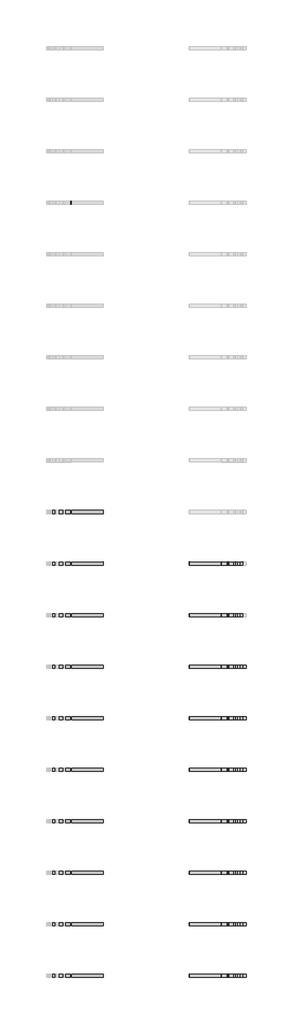
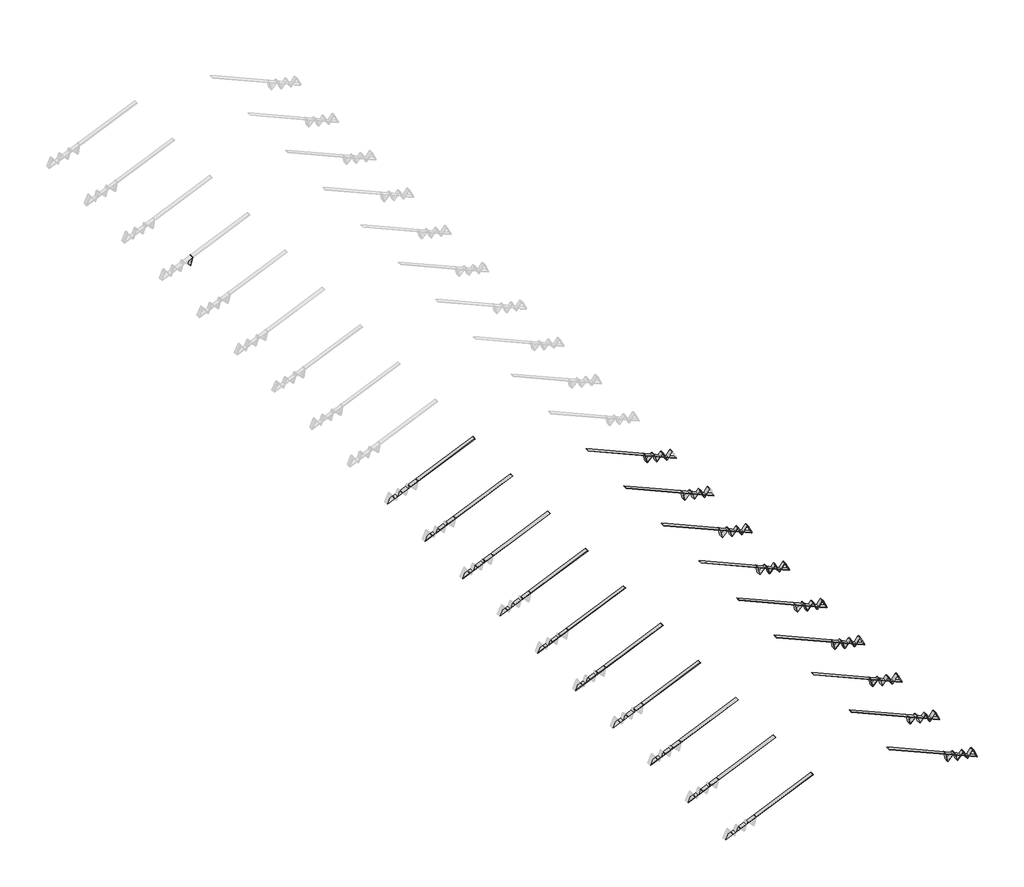
# One storey, part 2 of 4: 81 beams.
"""IFC4 building model written with IfcOpenShell, lengths in millimetres."""

import ifcopenshell
import ifcopenshell.guid

model = None  # the IFC model being written
_history = None  # IfcOwnerHistory: only IFC2X3 demands one
_inside = {}  # id of a spatial element -> (the spatial element, [elements in it])
_under = {}  # id of a project, library or spatial element -> (it, [spatial elements below it])
_declared = {}  # id of a project -> (the project, [libraries it declares])
_typed = {}  # id of a type object -> (the type object, [elements of that type])
_made_of = {}  # id of a material, layer set ... -> (it, [elements and type objects made of it])


def new_model(schema):
    """Start an empty IFC model of exactly this schema.

    Asked for "IFC4X3", IfcOpenShell would pick the latest addendum, in which some entities
    have other attributes; the version numbers below select the first issue.
    IFC2X3 requires an IfcOwnerHistory on every rooted entity: one is made here for all.
    """
    global model, _history
    if schema == "IFC4X3":
        model = ifcopenshell.file(schema_version=(4, 3, 0, 0))
    else:
        model = ifcopenshell.file(schema=schema)
    _inside.clear()
    _under.clear()
    _declared.clear()
    _typed.clear()
    _made_of.clear()
    _history = None
    if model.schema == "IFC2X3":
        org = make("IfcOrganization", Name="unknown")
        user = make(
            "IfcPersonAndOrganization",
            ThePerson=make("IfcPerson", FamilyName="unknown"),
            TheOrganization=org,
        )
        app = make(
            "IfcApplication",
            ApplicationDeveloper=org,
            Version="unknown",
            ApplicationFullName="unknown",
            ApplicationIdentifier="unknown",
        )
        _history = make(
            "IfcOwnerHistory",
            OwningUser=user,
            OwningApplication=app,
            ChangeAction="ADDED",
            CreationDate=0,
        )
    return model


def make(cls, **values):
    """One entity of the class cls with the attributes given. An attribute that is None is left unset."""
    return model.create_entity(
        cls, **{name: value for name, value in values.items() if value is not None}
    )


def rooted(cls, **values):
    """An entity with a GlobalId (a new one), such as an element, a storey or a relation."""
    return make(cls, GlobalId=ifcopenshell.guid.new(), OwnerHistory=_history, **values)


def si_unit(unit_type, name, prefix=None):
    """IfcSIUnit, for example si_unit("LENGTHUNIT", "METRE", prefix="MILLI")."""
    return make("IfcSIUnit", UnitType=unit_type, Prefix=prefix, Name=name)


def assignment(units):
    """IfcUnitAssignment: the units of a project."""
    return None if units is None else make("IfcUnitAssignment", Units=units)


def point(xyz):
    """IfcCartesianPoint."""
    return None if xyz is None else make("IfcCartesianPoint", Coordinates=xyz)


def direction(xyz):
    """IfcDirection."""
    return None if xyz is None else make("IfcDirection", DirectionRatios=xyz)


def frame(location, z_axis=None, x_axis=None):
    """IfcAxis2Placement3D, a coordinate frame: its origin and axes. An axis left out is left unset."""
    return make(
        "IfcAxis2Placement3D",
        Location=point(location),
        Axis=direction(z_axis),
        RefDirection=direction(x_axis),
    )


def frame_2d(location, x_axis=None):
    """IfcAxis2Placement2D, a coordinate frame in the plane: its origin and x axis."""
    return make(
        "IfcAxis2Placement2D", Location=point(location), RefDirection=direction(x_axis)
    )


def origin():
    """The frame at (0, 0, 0) with its axes left unset."""
    return frame((0.0, 0.0, 0.0))


def place(relative_to, where):
    """IfcLocalPlacement: puts the frame where relative to a parent placement (None: the world)."""
    return make(
        "IfcLocalPlacement", PlacementRelTo=relative_to, RelativePlacement=where
    )


def context(
    kind, dimensions, precision=None, world=None, true_north=None, identifier=None
):
    """IfcGeometricRepresentationContext, for example the 3D "Model" context."""
    return make(
        "IfcGeometricRepresentationContext",
        ContextIdentifier=identifier,
        ContextType=kind,
        CoordinateSpaceDimension=dimensions,
        Precision=precision,
        WorldCoordinateSystem=world,
        TrueNorth=true_north,
    )


def project(units=None, contexts=None):
    """IfcProject with its units and contexts."""
    return rooted(
        "IfcProject",
        Name="project",
        RepresentationContexts=contexts,
        UnitsInContext=assignment(units),
    )


def spatial(cls, under=None, at=None, **own):
    """A site, building, storey or space (cls), placed at a placement, below another one or the project."""
    s = rooted(cls, ObjectPlacement=at, **own)
    if under is not None:
        _under.setdefault(under.id(), (under, []))[1].append(s)
    return s


def polyline(points):
    """IfcPolyline through the points."""
    return make("IfcPolyline", Points=[point(p) for p in points])


def circle_curve(where, radius):
    """IfcCircle in the frame where."""
    return make("IfcCircle", Position=where, Radius=radius)


def trimmed(basis, trim1, trim2, sense, master):
    """IfcTrimmedCurve: the piece of a basis curve between two trims."""
    return make(
        "IfcTrimmedCurve",
        BasisCurve=basis,
        Trim1=trim1,
        Trim2=trim2,
        SenseAgreement=sense,
        MasterRepresentation=master,
    )


def segment(curve, same_sense, transition):
    """IfcCompositeCurveSegment."""
    return make(
        "IfcCompositeCurveSegment",
        Transition=transition,
        SameSense=same_sense,
        ParentCurve=curve,
    )


def composite_curve(segments, self_intersect=None):
    """IfcCompositeCurve: segments joined end to end."""
    return make("IfcCompositeCurve", Segments=segments, SelfIntersect=self_intersect)


def outline(outer, holes=None, kind="AREA"):
    """IfcArbitraryClosedProfileDef: a profile drawn as a closed curve; with holes, ...WithVoids."""
    if holes is None:
        return make("IfcArbitraryClosedProfileDef", ProfileType=kind, OuterCurve=outer)
    return make(
        "IfcArbitraryProfileDefWithVoids",
        ProfileType=kind,
        OuterCurve=outer,
        InnerCurves=holes,
    )


def extrude(swept, where, along, depth):
    """IfcExtrudedAreaSolid: the profile swept, set in the frame where, extruded along a direction by depth."""
    return make(
        "IfcExtrudedAreaSolid",
        SweptArea=swept,
        Position=where,
        ExtrudedDirection=direction(along),
        Depth=depth,
    )


def shape(context_of_items, identifier, shape_type, items):
    """IfcShapeRepresentation: the items that make up one representation, for example the "Body"."""
    return make(
        "IfcShapeRepresentation",
        ContextOfItems=context_of_items,
        RepresentationIdentifier=identifier,
        RepresentationType=shape_type,
        Items=items,
    )


def source(mapping_origin, context_of_items, identifier, shape_type, items):
    """IfcRepresentationMap: a shape defined once, which mapped items show again and again."""
    return make(
        "IfcRepresentationMap",
        MappingOrigin=mapping_origin,
        MappedRepresentation=shape(context_of_items, identifier, shape_type, items),
    )


def transform(
    local_origin,
    x_axis=None,
    y_axis=None,
    z_axis=None,
    scale=None,
    scale2=None,
    scale3=None,
    uniform=True,
):
    """IfcCartesianTransformationOperator3D, or its non-uniform kind. x_axis, y_axis, z_axis: its Axis1, 2, 3."""
    if uniform:
        return make(
            "IfcCartesianTransformationOperator3D",
            Axis1=direction(x_axis),
            Axis2=direction(y_axis),
            LocalOrigin=point(local_origin),
            Scale=scale,
            Axis3=direction(z_axis),
        )
    return make(
        "IfcCartesianTransformationOperator3DnonUniform",
        Axis1=direction(x_axis),
        Axis2=direction(y_axis),
        LocalOrigin=point(local_origin),
        Scale=scale,
        Axis3=direction(z_axis),
        Scale2=scale2,
        Scale3=scale3,
    )


def mapped(mapping_source, mapping_target):
    """IfcMappedItem: shows the shape of a source again, moved by a transform."""
    return make(
        "IfcMappedItem", MappingSource=mapping_source, MappingTarget=mapping_target
    )


def made_of(thing, what):
    """Note that an element or type object is made of a material, layer set ...; save() writes the relation."""
    if what is not None:
        _made_of.setdefault(what.id(), (what, []))[1].append(thing)
    return thing


def element(
    cls,
    number,
    at=None,
    inside=None,
    cuts=None,
    type_object=None,
    material=None,
    context=None,
    identifier="Body",
    shape_type=None,
    held_by="IfcProductDefinitionShape",
    body=None,
    shapes=None,
    **own,
):
    """One element of the class cls, such as IfcWall. Its Tag is "e" and its number.

    at: its placement. inside: the storey or other place that contains it. cuts: it is an
    opening in that element (IfcRelVoidsElement). A single representation is given by context,
    identifier, shape_type and body (its items); several are given by shapes. held_by: the class
    of the entity that holds the representations. save() writes the other relations.
    """
    e = rooted(cls, Tag="e%d" % number, ObjectPlacement=at, **own)
    if body is not None:
        shapes = [shape(context, identifier, shape_type, body)]
    if shapes is not None:
        e.Representation = make(held_by, Representations=shapes)
    if inside is not None:
        _inside.setdefault(inside.id(), (inside, []))[1].append(e)
    if cuts is not None:
        rooted(
            "IfcRelVoidsElement", RelatingBuildingElement=cuts, RelatedOpeningElement=e
        )
    if type_object is not None:
        _typed.setdefault(type_object.id(), (type_object, []))[1].append(e)
    return made_of(e, material)


def aggregate(whole, parts):
    """IfcRelAggregates: a whole, such as a stair, and the parts it consists of."""
    return rooted("IfcRelAggregates", RelatingObject=whole, RelatedObjects=parts)


def save(model, path):
    """Write the relations noted so far, then the file.

    IfcRelAggregates (storeys below a building ...), IfcRelContainedInSpatialStructure (elements
    in a storey), IfcRelDefinesByType, IfcRelAssociatesMaterial and IfcRelDeclares: one each for
    every whole, place, type object, material and project.
    """
    for whole, parts in _under.values():
        aggregate(whole, parts)
    for where, things in _inside.values():
        rooted(
            "IfcRelContainedInSpatialStructure",
            RelatedElements=things,
            RelatingStructure=where,
        )
    for kind, things in _typed.values():
        rooted("IfcRelDefinesByType", RelatedObjects=things, RelatingType=kind)
    for what, things in _made_of.values():
        rooted("IfcRelAssociatesMaterial", RelatedObjects=things, RelatingMaterial=what)
    for by, libraries in _declared.values():
        rooted("IfcRelDeclares", RelatingContext=by, RelatedDefinitions=libraries)
    model.write(path)


def placa_diagonal_af2a04a3(model_context):
    return source(origin(), model_context, "Body", "SweptSolid", [
        extrude(outline(polyline([(165.1705216, 75.0), (165.1705216, -75.0), (-165.4962729, -75.0), (-165.4962729, 75.0), (165.1705216, 75.0)])), frame((0.0, 0.0, -4.0), z_axis=(0.0, 0.0, 1.0), x_axis=(1.0, 0.0, 0.0)), (0.0, 0.0, 1.0), 8.0),
    ])


def placa_diagonal_6d03bdc5(model_context):
    return source(origin(), model_context, "Body", "SweptSolid", [
        extrude(outline(polyline([(191.209825, 75.0), (191.209825, -75.0), (-166.9394885, -75.0), (-166.9394885, 75.0), (191.209825, 75.0)])), frame((0.0, 0.0, -4.0), z_axis=(0.0, 0.0, 1.0), x_axis=(1.0, 0.0, 0.0)), (0.0, 0.0, 1.0), 8.0),
    ])


def placa_diagonal_30fa4039(model_context):
    return source(origin(), model_context, "Body", "SweptSolid", [
        extrude(outline(polyline([(167.0675386, 75.0), (167.0675386, -75.0), (-167.4240159, -75.0), (-167.4240159, 75.0), (167.0675386, 75.0)])), frame((0.0, 0.0, -4.0), z_axis=(0.0, 0.0, 1.0), x_axis=(1.0, 0.0, 0.0)), (0.0, 0.0, 1.0), 8.0),
    ])


def placa_diagonal_ded414cc(model_context):
    return source(origin(), model_context, "Body", "SweptSolid", [
        extrude(outline(polyline([(167.4240165, 75.0), (167.4240165, -75.0), (-167.0675392, -75.0), (-167.0675392, 75.0), (167.4240165, 75.0)])), frame((0.0, 0.0, -4.0), z_axis=(0.0, 0.0, 1.0), x_axis=(1.0, 0.0, 0.0)), (0.0, 0.0, 1.0), 8.0),
    ])


def placa_diagonal_4690b74a(model_context):
    return source(origin(), model_context, "Body", "SweptSolid", [
        extrude(outline(polyline([(167.0675389, 75.0), (167.0675389, -75.0), (-167.4240162, -75.0), (-167.4240162, 75.0), (167.0675389, 75.0)])), frame((0.0, 0.0, -4.0), z_axis=(0.0, 0.0, 1.0), x_axis=(1.0, 0.0, 0.0)), (0.0, 0.0, 1.0), 8.0),
    ])


def placa_diagonal_aaf0c3b6(model_context):
    return source(origin(), model_context, "Body", "SweptSolid", [
        extrude(outline(polyline([(167.4240163, 75.0), (167.4240163, -75.0), (-167.067539, -75.0), (-167.067539, 75.0), (167.4240163, 75.0)])), frame((0.0, 0.0, -4.0), z_axis=(0.0, 0.0, 1.0), x_axis=(1.0, 0.0, 0.0)), (0.0, 0.0, 1.0), 8.0),
    ])


model = new_model("IFC4")

# Units and contexts
model_context = context("Model", 3, world=origin())
ifc_project = project(units=[si_unit("LENGTHUNIT", "METRE", prefix="MILLI")], contexts=[model_context])

# Site, building, storey
site = spatial("IfcSite", under=ifc_project)
building = spatial("IfcBuilding", under=site)
storey = spatial("IfcBuildingStorey", under=building, Name="Nível 4", Elevation=48165.0)

# Beams
placement = place(None, origin())
element("IfcBeam", 1, ObjectType="Placa : banzo", at=placement, inside=storey, context=model_context, shape_type="SweptSolid", body=[
    extrude(outline(composite_curve([segment(polyline([(48158.5516223, 8114.9704041), (48174.5198715, 8115.9778843)]), True, "CONTINUOUS"), segment(trimmed(circle_curve(frame_2d((53506.1312788, 8452.3636953)), 5342.2126139), [point((48174.5198715, 8115.9778843))], [point((49646.1683419, 4759.1372282))], True, "CARTESIAN"), True, "CONTINUOUS"), segment(polyline([(49646.1683419, 4759.1372282), (49634.6077, 4748.0759643)]), True, "CONTINUOUS"), segment(trimmed(circle_curve(frame_2d((53506.1312788, 8452.3636953)), 5358.2126139), [point((49634.6077, 4748.0759643))], [point((48158.5516223, 8114.9704041))], False, "CARTESIAN"), True, "CONTINUOUS")], self_intersect=False)), frame((0.0, -39678.5623634, 0.0), z_axis=(0.0, 1.0, 0.0), x_axis=(0.0, 0.0, 1.0)), (0.0, 0.0, 1.0), 150.0),
])
element("IfcBeam", 2, ObjectType="Placa : banzo", at=placement, inside=storey, context=model_context, shape_type="SweptSolid", body=[
    extrude(outline(composite_curve([segment(polyline([(49634.6077, 1843.8240278), (49646.1683419, 1832.762764)]), True, "CONTINUOUS"), segment(trimmed(circle_curve(frame_2d((53506.1312788, -1860.4637031)), 5342.2126139), [point((49646.1683419, 1832.762764))], [point((48174.5198715, -1524.0778921))], True, "CARTESIAN"), True, "CONTINUOUS"), segment(polyline([(48174.5198715, -1524.0778921), (48158.5516223, -1523.070412)]), True, "CONTINUOUS"), segment(trimmed(circle_curve(frame_2d((53506.1312788, -1860.4637031)), 5358.2126139), [point((48158.5516223, -1523.070412))], [point((49634.6077, 1843.8240278))], False, "CARTESIAN"), True, "CONTINUOUS")], self_intersect=False)), frame((0.0, -39678.5623634, 0.0), z_axis=(0.0, 1.0, 0.0), x_axis=(0.0, 0.0, 1.0)), (0.0, 0.0, 1.0), 150.0),
])
element("IfcBeam", 3, ObjectType="Placa : banzo", at=placement, inside=storey, context=model_context, shape_type="SweptSolid", body=[
    extrude(outline(composite_curve([segment(polyline([(49634.6077, 1843.8240278), (49646.1683419, 1832.762764)]), True, "CONTINUOUS"), segment(trimmed(circle_curve(frame_2d((53506.1312788, -1860.4637031)), 5342.2126139), [point((49646.1683419, 1832.762764))], [point((48174.5198715, -1524.0778921))], True, "CARTESIAN"), True, "CONTINUOUS"), segment(polyline([(48174.5198715, -1524.0778921), (48158.5516223, -1523.070412)]), True, "CONTINUOUS"), segment(trimmed(circle_curve(frame_2d((53506.1312788, -1860.4637031)), 5358.2126139), [point((48158.5516223, -1523.070412))], [point((49634.6077, 1843.8240278))], False, "CARTESIAN"), True, "CONTINUOUS")], self_intersect=False)), frame((0.0, -17178.5623634, 0.0), z_axis=(0.0, 1.0, 0.0), x_axis=(0.0, 0.0, 1.0)), (0.0, 0.0, 1.0), 150.0),
])
element("IfcBeam", 4, ObjectType="Placa : banzo", at=placement, inside=storey, context=model_context, shape_type="SweptSolid", body=[
    extrude(outline(composite_curve([segment(polyline([(48158.5516223, 8114.9704041), (48174.5198715, 8115.9778843)]), True, "CONTINUOUS"), segment(trimmed(circle_curve(frame_2d((53506.1312788, 8452.3636953)), 5342.2126139), [point((48174.5198715, 8115.9778843))], [point((49646.1683419, 4759.1372282))], True, "CARTESIAN"), True, "CONTINUOUS"), segment(polyline([(49646.1683419, 4759.1372282), (49634.6077, 4748.0759643)]), True, "CONTINUOUS"), segment(trimmed(circle_curve(frame_2d((53506.1312788, 8452.3636953)), 5358.2126139), [point((49634.6077, 4748.0759643))], [point((48158.5516223, 8114.9704041))], False, "CARTESIAN"), True, "CONTINUOUS")], self_intersect=False)), frame((0.0, -19678.5623634, 0.0), z_axis=(0.0, 1.0, 0.0), x_axis=(0.0, 0.0, 1.0)), (0.0, 0.0, 1.0), 150.0),
])
element("IfcBeam", 5, ObjectType="Placa : banzo", at=placement, inside=storey, context=model_context, shape_type="SweptSolid", body=[
    extrude(outline(composite_curve([segment(polyline([(49634.6077, 1843.8240278), (49646.1683419, 1832.762764)]), True, "CONTINUOUS"), segment(trimmed(circle_curve(frame_2d((53506.1312788, -1860.4637031)), 5342.2126139), [point((49646.1683419, 1832.762764))], [point((48174.5198715, -1524.0778921))], True, "CARTESIAN"), True, "CONTINUOUS"), segment(polyline([(48174.5198715, -1524.0778921), (48158.5516223, -1523.070412)]), True, "CONTINUOUS"), segment(trimmed(circle_curve(frame_2d((53506.1312788, -1860.4637031)), 5358.2126139), [point((48158.5516223, -1523.070412))], [point((49634.6077, 1843.8240278))], False, "CARTESIAN"), True, "CONTINUOUS")], self_intersect=False)), frame((0.0, -19678.5623634, 0.0), z_axis=(0.0, 1.0, 0.0), x_axis=(0.0, 0.0, 1.0)), (0.0, 0.0, 1.0), 150.0),
])
element("IfcBeam", 6, ObjectType="Placa : banzo", at=placement, inside=storey, context=model_context, shape_type="SweptSolid", body=[
    extrude(outline(composite_curve([segment(polyline([(48158.5516223, 8114.9704041), (48174.5198715, 8115.9778843)]), True, "CONTINUOUS"), segment(trimmed(circle_curve(frame_2d((53506.1312788, 8452.3636953)), 5342.2126139), [point((48174.5198715, 8115.9778843))], [point((49646.1683419, 4759.1372282))], True, "CARTESIAN"), True, "CONTINUOUS"), segment(polyline([(49646.1683419, 4759.1372282), (49634.6077, 4748.0759643)]), True, "CONTINUOUS"), segment(trimmed(circle_curve(frame_2d((53506.1312788, 8452.3636953)), 5358.2126139), [point((49634.6077, 4748.0759643))], [point((48158.5516223, 8114.9704041))], False, "CARTESIAN"), True, "CONTINUOUS")], self_intersect=False)), frame((0.0, -22178.5623634, 0.0), z_axis=(0.0, 1.0, 0.0), x_axis=(0.0, 0.0, 1.0)), (0.0, 0.0, 1.0), 150.0),
])
element("IfcBeam", 7, ObjectType="Placa : banzo", at=placement, inside=storey, context=model_context, shape_type="SweptSolid", body=[
    extrude(outline(composite_curve([segment(polyline([(49634.6077, 1843.8240278), (49646.1683419, 1832.762764)]), True, "CONTINUOUS"), segment(trimmed(circle_curve(frame_2d((53506.1312788, -1860.4637031)), 5342.2126139), [point((49646.1683419, 1832.762764))], [point((48174.5198715, -1524.0778921))], True, "CARTESIAN"), True, "CONTINUOUS"), segment(polyline([(48174.5198715, -1524.0778921), (48158.5516223, -1523.070412)]), True, "CONTINUOUS"), segment(trimmed(circle_curve(frame_2d((53506.1312788, -1860.4637031)), 5358.2126139), [point((48158.5516223, -1523.070412))], [point((49634.6077, 1843.8240278))], False, "CARTESIAN"), True, "CONTINUOUS")], self_intersect=False)), frame((0.0, -22178.5623634, 0.0), z_axis=(0.0, 1.0, 0.0), x_axis=(0.0, 0.0, 1.0)), (0.0, 0.0, 1.0), 150.0),
])
element("IfcBeam", 8, ObjectType="Placa : banzo", at=placement, inside=storey, context=model_context, shape_type="SweptSolid", body=[
    extrude(outline(composite_curve([segment(polyline([(48158.5516223, 8114.9704041), (48174.5198715, 8115.9778843)]), True, "CONTINUOUS"), segment(trimmed(circle_curve(frame_2d((53506.1312788, 8452.3636953)), 5342.2126139), [point((48174.5198715, 8115.9778843))], [point((49646.1683419, 4759.1372282))], True, "CARTESIAN"), True, "CONTINUOUS"), segment(polyline([(49646.1683419, 4759.1372282), (49634.6077, 4748.0759643)]), True, "CONTINUOUS"), segment(trimmed(circle_curve(frame_2d((53506.1312788, 8452.3636953)), 5358.2126139), [point((49634.6077, 4748.0759643))], [point((48158.5516223, 8114.9704041))], False, "CARTESIAN"), True, "CONTINUOUS")], self_intersect=False)), frame((0.0, -24678.5623634, 0.0), z_axis=(0.0, 1.0, 0.0), x_axis=(0.0, 0.0, 1.0)), (0.0, 0.0, 1.0), 150.0),
])
element("IfcBeam", 9, ObjectType="Placa : banzo", at=placement, inside=storey, context=model_context, shape_type="SweptSolid", body=[
    extrude(outline(composite_curve([segment(polyline([(49634.6077, 1843.8240278), (49646.1683419, 1832.762764)]), True, "CONTINUOUS"), segment(trimmed(circle_curve(frame_2d((53506.1312788, -1860.4637031)), 5342.2126139), [point((49646.1683419, 1832.762764))], [point((48174.5198715, -1524.0778921))], True, "CARTESIAN"), True, "CONTINUOUS"), segment(polyline([(48174.5198715, -1524.0778921), (48158.5516223, -1523.070412)]), True, "CONTINUOUS"), segment(trimmed(circle_curve(frame_2d((53506.1312788, -1860.4637031)), 5358.2126139), [point((48158.5516223, -1523.070412))], [point((49634.6077, 1843.8240278))], False, "CARTESIAN"), True, "CONTINUOUS")], self_intersect=False)), frame((0.0, -24678.5623634, 0.0), z_axis=(0.0, 1.0, 0.0), x_axis=(0.0, 0.0, 1.0)), (0.0, 0.0, 1.0), 150.0),
])
element("IfcBeam", 10, ObjectType="Placa : banzo", at=placement, inside=storey, context=model_context, shape_type="SweptSolid", body=[
    extrude(outline(composite_curve([segment(polyline([(48158.5516223, 8114.9704041), (48174.5198715, 8115.9778843)]), True, "CONTINUOUS"), segment(trimmed(circle_curve(frame_2d((53506.1312788, 8452.3636953)), 5342.2126139), [point((48174.5198715, 8115.9778843))], [point((49646.1683419, 4759.1372282))], True, "CARTESIAN"), True, "CONTINUOUS"), segment(polyline([(49646.1683419, 4759.1372282), (49634.6077, 4748.0759643)]), True, "CONTINUOUS"), segment(trimmed(circle_curve(frame_2d((53506.1312788, 8452.3636953)), 5358.2126139), [point((49634.6077, 4748.0759643))], [point((48158.5516223, 8114.9704041))], False, "CARTESIAN"), True, "CONTINUOUS")], self_intersect=False)), frame((0.0, -27178.5623634, 0.0), z_axis=(0.0, 1.0, 0.0), x_axis=(0.0, 0.0, 1.0)), (0.0, 0.0, 1.0), 150.0),
])
element("IfcBeam", 11, ObjectType="Placa : banzo", at=placement, inside=storey, context=model_context, shape_type="SweptSolid", body=[
    extrude(outline(composite_curve([segment(polyline([(49634.6077, 1843.8240278), (49646.1683419, 1832.762764)]), True, "CONTINUOUS"), segment(trimmed(circle_curve(frame_2d((53506.1312788, -1860.4637031)), 5342.2126139), [point((49646.1683419, 1832.762764))], [point((48174.5198715, -1524.0778921))], True, "CARTESIAN"), True, "CONTINUOUS"), segment(polyline([(48174.5198715, -1524.0778921), (48158.5516223, -1523.070412)]), True, "CONTINUOUS"), segment(trimmed(circle_curve(frame_2d((53506.1312788, -1860.4637031)), 5358.2126139), [point((48158.5516223, -1523.070412))], [point((49634.6077, 1843.8240278))], False, "CARTESIAN"), True, "CONTINUOUS")], self_intersect=False)), frame((0.0, -27178.5623634, 0.0), z_axis=(0.0, 1.0, 0.0), x_axis=(0.0, 0.0, 1.0)), (0.0, 0.0, 1.0), 150.0),
])
element("IfcBeam", 12, ObjectType="Placa : banzo", at=placement, inside=storey, context=model_context, shape_type="SweptSolid", body=[
    extrude(outline(composite_curve([segment(polyline([(48158.5516223, 8114.9704041), (48174.5198715, 8115.9778843)]), True, "CONTINUOUS"), segment(trimmed(circle_curve(frame_2d((53506.1312788, 8452.3636953)), 5342.2126139), [point((48174.5198715, 8115.9778843))], [point((49646.1683419, 4759.1372282))], True, "CARTESIAN"), True, "CONTINUOUS"), segment(polyline([(49646.1683419, 4759.1372282), (49634.6077, 4748.0759643)]), True, "CONTINUOUS"), segment(trimmed(circle_curve(frame_2d((53506.1312788, 8452.3636953)), 5358.2126139), [point((49634.6077, 4748.0759643))], [point((48158.5516223, 8114.9704041))], False, "CARTESIAN"), True, "CONTINUOUS")], self_intersect=False)), frame((0.0, -29678.5623634, 0.0), z_axis=(0.0, 1.0, 0.0), x_axis=(0.0, 0.0, 1.0)), (0.0, 0.0, 1.0), 150.0),
])
element("IfcBeam", 13, ObjectType="Placa : banzo", at=placement, inside=storey, context=model_context, shape_type="SweptSolid", body=[
    extrude(outline(composite_curve([segment(polyline([(49634.6077, 1843.8240278), (49646.1683419, 1832.762764)]), True, "CONTINUOUS"), segment(trimmed(circle_curve(frame_2d((53506.1312788, -1860.4637031)), 5342.2126139), [point((49646.1683419, 1832.762764))], [point((48174.5198715, -1524.0778921))], True, "CARTESIAN"), True, "CONTINUOUS"), segment(polyline([(48174.5198715, -1524.0778921), (48158.5516223, -1523.070412)]), True, "CONTINUOUS"), segment(trimmed(circle_curve(frame_2d((53506.1312788, -1860.4637031)), 5358.2126139), [point((48158.5516223, -1523.070412))], [point((49634.6077, 1843.8240278))], False, "CARTESIAN"), True, "CONTINUOUS")], self_intersect=False)), frame((0.0, -29678.5623634, 0.0), z_axis=(0.0, 1.0, 0.0), x_axis=(0.0, 0.0, 1.0)), (0.0, 0.0, 1.0), 150.0),
])
element("IfcBeam", 14, ObjectType="Placa : banzo", at=placement, inside=storey, context=model_context, shape_type="SweptSolid", body=[
    extrude(outline(composite_curve([segment(polyline([(48158.5516223, 8114.9704041), (48174.5198715, 8115.9778843)]), True, "CONTINUOUS"), segment(trimmed(circle_curve(frame_2d((53506.1312788, 8452.3636953)), 5342.2126139), [point((48174.5198715, 8115.9778843))], [point((49646.1683419, 4759.1372282))], True, "CARTESIAN"), True, "CONTINUOUS"), segment(polyline([(49646.1683419, 4759.1372282), (49634.6077, 4748.0759643)]), True, "CONTINUOUS"), segment(trimmed(circle_curve(frame_2d((53506.1312788, 8452.3636953)), 5358.2126139), [point((49634.6077, 4748.0759643))], [point((48158.5516223, 8114.9704041))], False, "CARTESIAN"), True, "CONTINUOUS")], self_intersect=False)), frame((0.0, -32178.5623634, 0.0), z_axis=(0.0, 1.0, 0.0), x_axis=(0.0, 0.0, 1.0)), (0.0, 0.0, 1.0), 150.0),
])
element("IfcBeam", 15, ObjectType="Placa : banzo", at=placement, inside=storey, context=model_context, shape_type="SweptSolid", body=[
    extrude(outline(composite_curve([segment(polyline([(49634.6077, 1843.8240278), (49646.1683419, 1832.762764)]), True, "CONTINUOUS"), segment(trimmed(circle_curve(frame_2d((53506.1312788, -1860.4637031)), 5342.2126139), [point((49646.1683419, 1832.762764))], [point((48174.5198715, -1524.0778921))], True, "CARTESIAN"), True, "CONTINUOUS"), segment(polyline([(48174.5198715, -1524.0778921), (48158.5516223, -1523.070412)]), True, "CONTINUOUS"), segment(trimmed(circle_curve(frame_2d((53506.1312788, -1860.4637031)), 5358.2126139), [point((48158.5516223, -1523.070412))], [point((49634.6077, 1843.8240278))], False, "CARTESIAN"), True, "CONTINUOUS")], self_intersect=False)), frame((0.0, -32178.5623634, 0.0), z_axis=(0.0, 1.0, 0.0), x_axis=(0.0, 0.0, 1.0)), (0.0, 0.0, 1.0), 150.0),
])
element("IfcBeam", 16, ObjectType="Placa : banzo", at=placement, inside=storey, context=model_context, shape_type="SweptSolid", body=[
    extrude(outline(composite_curve([segment(polyline([(48158.5516223, 8114.9704041), (48174.5198715, 8115.9778843)]), True, "CONTINUOUS"), segment(trimmed(circle_curve(frame_2d((53506.1312788, 8452.3636953)), 5342.2126139), [point((48174.5198715, 8115.9778843))], [point((49646.1683419, 4759.1372282))], True, "CARTESIAN"), True, "CONTINUOUS"), segment(polyline([(49646.1683419, 4759.1372282), (49634.6077, 4748.0759643)]), True, "CONTINUOUS"), segment(trimmed(circle_curve(frame_2d((53506.1312788, 8452.3636953)), 5358.2126139), [point((49634.6077, 4748.0759643))], [point((48158.5516223, 8114.9704041))], False, "CARTESIAN"), True, "CONTINUOUS")], self_intersect=False)), frame((0.0, -34678.5623634, 0.0), z_axis=(0.0, 1.0, 0.0), x_axis=(0.0, 0.0, 1.0)), (0.0, 0.0, 1.0), 150.0),
])
element("IfcBeam", 17, ObjectType="Placa : banzo", at=placement, inside=storey, context=model_context, shape_type="SweptSolid", body=[
    extrude(outline(composite_curve([segment(polyline([(49634.6077, 1843.8240278), (49646.1683419, 1832.762764)]), True, "CONTINUOUS"), segment(trimmed(circle_curve(frame_2d((53506.1312788, -1860.4637031)), 5342.2126139), [point((49646.1683419, 1832.762764))], [point((48174.5198715, -1524.0778921))], True, "CARTESIAN"), True, "CONTINUOUS"), segment(polyline([(48174.5198715, -1524.0778921), (48158.5516223, -1523.070412)]), True, "CONTINUOUS"), segment(trimmed(circle_curve(frame_2d((53506.1312788, -1860.4637031)), 5358.2126139), [point((48158.5516223, -1523.070412))], [point((49634.6077, 1843.8240278))], False, "CARTESIAN"), True, "CONTINUOUS")], self_intersect=False)), frame((0.0, -34678.5623634, 0.0), z_axis=(0.0, 1.0, 0.0), x_axis=(0.0, 0.0, 1.0)), (0.0, 0.0, 1.0), 150.0),
])
element("IfcBeam", 18, ObjectType="Placa : banzo", at=placement, inside=storey, context=model_context, shape_type="SweptSolid", body=[
    extrude(outline(composite_curve([segment(polyline([(48158.5516223, 8114.9704041), (48174.5198715, 8115.9778843)]), True, "CONTINUOUS"), segment(trimmed(circle_curve(frame_2d((53506.1312788, 8452.3636953)), 5342.2126139), [point((48174.5198715, 8115.9778843))], [point((49646.1683419, 4759.1372282))], True, "CARTESIAN"), True, "CONTINUOUS"), segment(polyline([(49646.1683419, 4759.1372282), (49634.6077, 4748.0759643)]), True, "CONTINUOUS"), segment(trimmed(circle_curve(frame_2d((53506.1312788, 8452.3636953)), 5358.2126139), [point((49634.6077, 4748.0759643))], [point((48158.5516223, 8114.9704041))], False, "CARTESIAN"), True, "CONTINUOUS")], self_intersect=False)), frame((0.0, -37178.5623634, 0.0), z_axis=(0.0, 1.0, 0.0), x_axis=(0.0, 0.0, 1.0)), (0.0, 0.0, 1.0), 150.0),
])
element("IfcBeam", 19, ObjectType="Placa : banzo", at=placement, inside=storey, context=model_context, shape_type="SweptSolid", body=[
    extrude(outline(composite_curve([segment(polyline([(49634.6077, 1843.8240278), (49646.1683419, 1832.762764)]), True, "CONTINUOUS"), segment(trimmed(circle_curve(frame_2d((53506.1312788, -1860.4637031)), 5342.2126139), [point((49646.1683419, 1832.762764))], [point((48174.5198715, -1524.0778921))], True, "CARTESIAN"), True, "CONTINUOUS"), segment(polyline([(48174.5198715, -1524.0778921), (48158.5516223, -1523.070412)]), True, "CONTINUOUS"), segment(trimmed(circle_curve(frame_2d((53506.1312788, -1860.4637031)), 5358.2126139), [point((48158.5516223, -1523.070412))], [point((49634.6077, 1843.8240278))], False, "CARTESIAN"), True, "CONTINUOUS")], self_intersect=False)), frame((0.0, -37178.5623634, 0.0), z_axis=(0.0, 1.0, 0.0), x_axis=(0.0, 0.0, 1.0)), (0.0, 0.0, 1.0), 150.0),
])
placa_diagonal_shape = placa_diagonal_af2a04a3(model_context)
element("IfcBeam", 20, ObjectType="Placa : diagonal", at=placement, inside=storey, context=model_context, shape_type="MappedRepresentation", body=[
    mapped(placa_diagonal_shape, transform((-392.7303205, -2103.5623634, 48535.8666224), x_axis=(0.20085127706480188, 0.0, 0.9796217456250337), y_axis=(0.0, -1.0, 0.0), z_axis=(0.9796217456250337, 0.0, -0.20085127706480188))),
])
placa_diagonal_2_shape = placa_diagonal_6d03bdc5(model_context)
element("IfcBeam", 21, ObjectType="Placa : diagonal", at=placement, inside=storey, context=model_context, shape_type="MappedRepresentation", body=[
    mapped(placa_diagonal_2_shape, transform((8059.7198757, -39603.5623634, 48338.6280973), x_axis=(0.4189773842608123, 0.0, -0.9079966693099526), y_axis=(0.0, -1.0, 0.0), z_axis=(-0.9079966693099526, 0.0, -0.4189773842608123))),
])
element("IfcBeam", 22, ObjectType="Placa : diagonal", at=placement, inside=storey, context=model_context, shape_type="MappedRepresentation", body=[
    mapped(placa_diagonal_2_shape, transform((8059.7198757, -24603.5623634, 48338.6280973), x_axis=(0.4189773842608123, 0.0, -0.9079966693099526), y_axis=(0.0, -1.0, 0.0), z_axis=(-0.9079966693099526, 0.0, -0.4189773842608123))),
])
element("IfcBeam", 23, ObjectType="Placa : diagonal", at=placement, inside=storey, context=model_context, shape_type="MappedRepresentation", body=[
    mapped(placa_diagonal_2_shape, transform((8059.7198757, -27103.5623634, 48338.6280973), x_axis=(0.4189773842608123, 0.0, -0.9079966693099526), y_axis=(0.0, -1.0, 0.0), z_axis=(-0.9079966693099526, 0.0, -0.4189773842608123))),
])
element("IfcBeam", 24, ObjectType="Placa : diagonal", at=placement, inside=storey, context=model_context, shape_type="MappedRepresentation", body=[
    mapped(placa_diagonal_2_shape, transform((8059.7198757, -29603.5623634, 48338.6280973), x_axis=(0.4189773842608123, 0.0, -0.9079966693099526), y_axis=(0.0, -1.0, 0.0), z_axis=(-0.9079966693099526, 0.0, -0.4189773842608123))),
])
element("IfcBeam", 25, ObjectType="Placa : diagonal", at=placement, inside=storey, context=model_context, shape_type="MappedRepresentation", body=[
    mapped(placa_diagonal_2_shape, transform((8059.7198757, -32103.5623634, 48338.6280973), x_axis=(0.4189773842608123, 0.0, -0.9079966693099526), y_axis=(0.0, -1.0, 0.0), z_axis=(-0.9079966693099526, 0.0, -0.4189773842608123))),
])
element("IfcBeam", 26, ObjectType="Placa : diagonal", at=placement, inside=storey, context=model_context, shape_type="MappedRepresentation", body=[
    mapped(placa_diagonal_2_shape, transform((8059.7198757, -34603.5623634, 48338.6280973), x_axis=(0.4189773842608123, 0.0, -0.9079966693099526), y_axis=(0.0, -1.0, 0.0), z_axis=(-0.9079966693099526, 0.0, -0.4189773842608123))),
])
element("IfcBeam", 27, ObjectType="Placa : diagonal", at=placement, inside=storey, context=model_context, shape_type="MappedRepresentation", body=[
    mapped(placa_diagonal_2_shape, transform((8059.7198757, -37103.5623634, 48338.6280973), x_axis=(0.4189773842608123, 0.0, -0.9079966693099526), y_axis=(0.0, -1.0, 0.0), z_axis=(-0.9079966693099526, 0.0, -0.4189773842608123))),
])
placa_diagonal_3_shape = placa_diagonal_30fa4039(model_context)
element("IfcBeam", 28, ObjectType="Placa : diagonal", at=placement, inside=storey, context=model_context, shape_type="MappedRepresentation", body=[
    mapped(placa_diagonal_3_shape, transform((7867.9931921, -39603.5623634, 48356.8132581), x_axis=(0.5832804616623758, 0.0, 0.8122708310920229), y_axis=(0.0, -1.0, 0.0), z_axis=(0.8122708310920229, 0.0, -0.5832804616623758))),
])
element("IfcBeam", 29, ObjectType="Placa : diagonal", at=placement, inside=storey, context=model_context, shape_type="MappedRepresentation", body=[
    mapped(placa_diagonal_3_shape, transform((7867.9931921, -19603.5623634, 48356.8132581), x_axis=(0.5832804616623758, 0.0, 0.8122708310920229), y_axis=(0.0, -1.0, 0.0), z_axis=(0.8122708310920229, 0.0, -0.5832804616623758))),
])
element("IfcBeam", 30, ObjectType="Placa : diagonal", at=placement, inside=storey, context=model_context, shape_type="MappedRepresentation", body=[
    mapped(placa_diagonal_3_shape, transform((7867.9931921, -22103.5623634, 48356.8132581), x_axis=(0.5832804616623758, 0.0, 0.8122708310920229), y_axis=(0.0, -1.0, 0.0), z_axis=(0.8122708310920229, 0.0, -0.5832804616623758))),
])
element("IfcBeam", 31, ObjectType="Placa : diagonal", at=placement, inside=storey, context=model_context, shape_type="MappedRepresentation", body=[
    mapped(placa_diagonal_3_shape, transform((7867.9931921, -24603.5623634, 48356.8132581), x_axis=(0.5832804616623758, 0.0, 0.8122708310920229), y_axis=(0.0, -1.0, 0.0), z_axis=(0.8122708310920229, 0.0, -0.5832804616623758))),
])
element("IfcBeam", 32, ObjectType="Placa : diagonal", at=placement, inside=storey, context=model_context, shape_type="MappedRepresentation", body=[
    mapped(placa_diagonal_3_shape, transform((7867.9931921, -27103.5623634, 48356.8132581), x_axis=(0.5832804616623758, 0.0, 0.8122708310920229), y_axis=(0.0, -1.0, 0.0), z_axis=(0.8122708310920229, 0.0, -0.5832804616623758))),
])
element("IfcBeam", 33, ObjectType="Placa : diagonal", at=placement, inside=storey, context=model_context, shape_type="MappedRepresentation", body=[
    mapped(placa_diagonal_3_shape, transform((7867.9931921, -29603.5623634, 48356.8132581), x_axis=(0.5832804616623758, 0.0, 0.8122708310920229), y_axis=(0.0, -1.0, 0.0), z_axis=(0.8122708310920229, 0.0, -0.5832804616623758))),
])
element("IfcBeam", 34, ObjectType="Placa : diagonal", at=placement, inside=storey, context=model_context, shape_type="MappedRepresentation", body=[
    mapped(placa_diagonal_3_shape, transform((7867.9931921, -32103.5623634, 48356.8132581), x_axis=(0.5832804616623758, 0.0, 0.8122708310920229), y_axis=(0.0, -1.0, 0.0), z_axis=(0.8122708310920229, 0.0, -0.5832804616623758))),
])
element("IfcBeam", 35, ObjectType="Placa : diagonal", at=placement, inside=storey, context=model_context, shape_type="MappedRepresentation", body=[
    mapped(placa_diagonal_3_shape, transform((7867.9931921, -34603.5623634, 48356.8132581), x_axis=(0.5832804616623758, 0.0, 0.8122708310920229), y_axis=(0.0, -1.0, 0.0), z_axis=(0.8122708310920229, 0.0, -0.5832804616623758))),
])
element("IfcBeam", 36, ObjectType="Placa : diagonal", at=placement, inside=storey, context=model_context, shape_type="MappedRepresentation", body=[
    mapped(placa_diagonal_3_shape, transform((7867.9931921, -37103.5623634, 48356.8132581), x_axis=(0.5832804616623758, 0.0, 0.8122708310920229), y_axis=(0.0, -1.0, 0.0), z_axis=(0.8122708310920229, 0.0, -0.5832804616623758))),
])
placa_diagonal_4_shape = placa_diagonal_ded414cc(model_context)
element("IfcBeam", 37, ObjectType="Placa : diagonal", at=placement, inside=storey, context=model_context, shape_type="MappedRepresentation", body=[
    mapped(placa_diagonal_4_shape, transform((7688.6379629, -39603.5623634, 48380.344708), x_axis=(0.3540062158971715, 0.0, -0.935243069531213), y_axis=(0.0, -1.0, 0.0), z_axis=(-0.935243069531213, 0.0, -0.3540062158971715))),
])
element("IfcBeam", 38, ObjectType="Placa : diagonal", at=placement, inside=storey, context=model_context, shape_type="MappedRepresentation", body=[
    mapped(placa_diagonal_4_shape, transform((7321.1773395, -39603.5623634, 48448.7226144), x_axis=(0.2856767726847757, 0.0, -0.9583260309249723), y_axis=(0.0, -1.0, 0.0), z_axis=(-0.9583260309249723, 0.0, -0.2856767726847757))),
])
element("IfcBeam", 39, ObjectType="Placa : diagonal", at=placement, inside=storey, context=model_context, shape_type="MappedRepresentation", body=[
    mapped(placa_diagonal_4_shape, transform((7688.6379629, -19603.5623634, 48380.344708), x_axis=(0.3540062158971715, 0.0, -0.935243069531213), y_axis=(0.0, -1.0, 0.0), z_axis=(-0.935243069531213, 0.0, -0.3540062158971715))),
])
element("IfcBeam", 40, ObjectType="Placa : diagonal", at=placement, inside=storey, context=model_context, shape_type="MappedRepresentation", body=[
    mapped(placa_diagonal_4_shape, transform((7321.1773395, -19603.5623634, 48448.7226144), x_axis=(0.2856767726847757, 0.0, -0.9583260309249723), y_axis=(0.0, -1.0, 0.0), z_axis=(-0.9583260309249723, 0.0, -0.2856767726847757))),
])
element("IfcBeam", 41, ObjectType="Placa : diagonal", at=placement, inside=storey, context=model_context, shape_type="MappedRepresentation", body=[
    mapped(placa_diagonal_4_shape, transform((7688.6379629, -22103.5623634, 48380.344708), x_axis=(0.3540062158971715, 0.0, -0.935243069531213), y_axis=(0.0, -1.0, 0.0), z_axis=(-0.935243069531213, 0.0, -0.3540062158971715))),
])
element("IfcBeam", 42, ObjectType="Placa : diagonal", at=placement, inside=storey, context=model_context, shape_type="MappedRepresentation", body=[
    mapped(placa_diagonal_4_shape, transform((7321.1773395, -22103.5623634, 48448.7226144), x_axis=(0.2856767726847757, 0.0, -0.9583260309249723), y_axis=(0.0, -1.0, 0.0), z_axis=(-0.9583260309249723, 0.0, -0.2856767726847757))),
])
element("IfcBeam", 43, ObjectType="Placa : diagonal", at=placement, inside=storey, context=model_context, shape_type="MappedRepresentation", body=[
    mapped(placa_diagonal_4_shape, transform((7688.6379629, -24603.5623634, 48380.344708), x_axis=(0.3540062158971715, 0.0, -0.935243069531213), y_axis=(0.0, -1.0, 0.0), z_axis=(-0.935243069531213, 0.0, -0.3540062158971715))),
])
element("IfcBeam", 44, ObjectType="Placa : diagonal", at=placement, inside=storey, context=model_context, shape_type="MappedRepresentation", body=[
    mapped(placa_diagonal_4_shape, transform((7321.1773395, -24603.5623634, 48448.7226144), x_axis=(0.2856767726847757, 0.0, -0.9583260309249723), y_axis=(0.0, -1.0, 0.0), z_axis=(-0.9583260309249723, 0.0, -0.2856767726847757))),
])
element("IfcBeam", 45, ObjectType="Placa : diagonal", at=placement, inside=storey, context=model_context, shape_type="MappedRepresentation", body=[
    mapped(placa_diagonal_4_shape, transform((7688.6379629, -27103.5623634, 48380.344708), x_axis=(0.3540062158971715, 0.0, -0.935243069531213), y_axis=(0.0, -1.0, 0.0), z_axis=(-0.935243069531213, 0.0, -0.3540062158971715))),
])
element("IfcBeam", 46, ObjectType="Placa : diagonal", at=placement, inside=storey, context=model_context, shape_type="MappedRepresentation", body=[
    mapped(placa_diagonal_4_shape, transform((7321.1773395, -27103.5623634, 48448.7226144), x_axis=(0.2856767726847757, 0.0, -0.9583260309249723), y_axis=(0.0, -1.0, 0.0), z_axis=(-0.9583260309249723, 0.0, -0.2856767726847757))),
])
element("IfcBeam", 47, ObjectType="Placa : diagonal", at=placement, inside=storey, context=model_context, shape_type="MappedRepresentation", body=[
    mapped(placa_diagonal_4_shape, transform((7688.6379629, -29603.5623634, 48380.344708), x_axis=(0.3540062158971715, 0.0, -0.935243069531213), y_axis=(0.0, -1.0, 0.0), z_axis=(-0.935243069531213, 0.0, -0.3540062158971715))),
])
element("IfcBeam", 48, ObjectType="Placa : diagonal", at=placement, inside=storey, context=model_context, shape_type="MappedRepresentation", body=[
    mapped(placa_diagonal_4_shape, transform((7321.1773395, -29603.5623634, 48448.7226144), x_axis=(0.2856767726847757, 0.0, -0.9583260309249723), y_axis=(0.0, -1.0, 0.0), z_axis=(-0.9583260309249723, 0.0, -0.2856767726847757))),
])
element("IfcBeam", 49, ObjectType="Placa : diagonal", at=placement, inside=storey, context=model_context, shape_type="MappedRepresentation", body=[
    mapped(placa_diagonal_4_shape, transform((7688.6379629, -32103.5623634, 48380.344708), x_axis=(0.3540062158971715, 0.0, -0.935243069531213), y_axis=(0.0, -1.0, 0.0), z_axis=(-0.935243069531213, 0.0, -0.3540062158971715))),
])
element("IfcBeam", 50, ObjectType="Placa : diagonal", at=placement, inside=storey, context=model_context, shape_type="MappedRepresentation", body=[
    mapped(placa_diagonal_4_shape, transform((7321.1773395, -32103.5623634, 48448.7226144), x_axis=(0.2856767726847757, 0.0, -0.9583260309249723), y_axis=(0.0, -1.0, 0.0), z_axis=(-0.9583260309249723, 0.0, -0.2856767726847757))),
])
element("IfcBeam", 51, ObjectType="Placa : diagonal", at=placement, inside=storey, context=model_context, shape_type="MappedRepresentation", body=[
    mapped(placa_diagonal_4_shape, transform((7688.6379629, -34603.5623634, 48380.344708), x_axis=(0.3540062158971715, 0.0, -0.935243069531213), y_axis=(0.0, -1.0, 0.0), z_axis=(-0.935243069531213, 0.0, -0.3540062158971715))),
])
element("IfcBeam", 52, ObjectType="Placa : diagonal", at=placement, inside=storey, context=model_context, shape_type="MappedRepresentation", body=[
    mapped(placa_diagonal_4_shape, transform((7321.1773395, -34603.5623634, 48448.7226144), x_axis=(0.2856767726847757, 0.0, -0.9583260309249723), y_axis=(0.0, -1.0, 0.0), z_axis=(-0.9583260309249723, 0.0, -0.2856767726847757))),
])
element("IfcBeam", 53, ObjectType="Placa : diagonal", at=placement, inside=storey, context=model_context, shape_type="MappedRepresentation", body=[
    mapped(placa_diagonal_4_shape, transform((7688.6379629, -37103.5623634, 48380.344708), x_axis=(0.3540062158971715, 0.0, -0.935243069531213), y_axis=(0.0, -1.0, 0.0), z_axis=(-0.935243069531213, 0.0, -0.3540062158971715))),
])
element("IfcBeam", 54, ObjectType="Placa : diagonal", at=placement, inside=storey, context=model_context, shape_type="MappedRepresentation", body=[
    mapped(placa_diagonal_4_shape, transform((7321.1773395, -37103.5623634, 48448.7226144), x_axis=(0.2856767726847757, 0.0, -0.9583260309249723), y_axis=(0.0, -1.0, 0.0), z_axis=(-0.9583260309249723, 0.0, -0.2856767726847757))),
])
placa_diagonal_5_shape = placa_diagonal_4690b74a(model_context)
element("IfcBeam", 55, ObjectType="Placa : diagonal", at=placement, inside=storey, context=model_context, shape_type="MappedRepresentation", body=[
    mapped(placa_diagonal_5_shape, transform((7498.370034, -39603.5623634, 48412.3251322), x_axis=(0.6403087836754673, 0.0, 0.7681176091901837), y_axis=(0.0, -1.0, 0.0), z_axis=(0.7681176091901837, 0.0, -0.6403087836754673))),
])
element("IfcBeam", 56, ObjectType="Placa : diagonal", at=placement, inside=storey, context=model_context, shape_type="MappedRepresentation", body=[
    mapped(placa_diagonal_5_shape, transform((7133.7092978, -39603.5623634, 48494.333642), x_axis=(0.6940063880716316, 0.0, 0.719968841906209), y_axis=(0.0, -1.0, 0.0), z_axis=(0.719968841906209, 0.0, -0.6940063880716316))),
])
element("IfcBeam", 57, ObjectType="Placa : diagonal", at=placement, inside=storey, context=model_context, shape_type="MappedRepresentation", body=[
    mapped(placa_diagonal_5_shape, transform((7498.370034, -19603.5623634, 48412.3251322), x_axis=(0.6403087836754673, 0.0, 0.7681176091901837), y_axis=(0.0, -1.0, 0.0), z_axis=(0.7681176091901837, 0.0, -0.6403087836754673))),
])
element("IfcBeam", 58, ObjectType="Placa : diagonal", at=placement, inside=storey, context=model_context, shape_type="MappedRepresentation", body=[
    mapped(placa_diagonal_5_shape, transform((7133.7092978, -19603.5623634, 48494.333642), x_axis=(0.6940063880716316, 0.0, 0.719968841906209), y_axis=(0.0, -1.0, 0.0), z_axis=(0.719968841906209, 0.0, -0.6940063880716316))),
])
element("IfcBeam", 59, ObjectType="Placa : diagonal", at=placement, inside=storey, context=model_context, shape_type="MappedRepresentation", body=[
    mapped(placa_diagonal_5_shape, transform((7498.370034, -22103.5623634, 48412.3251322), x_axis=(0.6403087836754673, 0.0, 0.7681176091901837), y_axis=(0.0, -1.0, 0.0), z_axis=(0.7681176091901837, 0.0, -0.6403087836754673))),
])
element("IfcBeam", 60, ObjectType="Placa : diagonal", at=placement, inside=storey, context=model_context, shape_type="MappedRepresentation", body=[
    mapped(placa_diagonal_5_shape, transform((7133.7092978, -22103.5623634, 48494.333642), x_axis=(0.6940063880716316, 0.0, 0.719968841906209), y_axis=(0.0, -1.0, 0.0), z_axis=(0.719968841906209, 0.0, -0.6940063880716316))),
])
element("IfcBeam", 61, ObjectType="Placa : diagonal", at=placement, inside=storey, context=model_context, shape_type="MappedRepresentation", body=[
    mapped(placa_diagonal_5_shape, transform((7498.370034, -24603.5623634, 48412.3251322), x_axis=(0.6403087836754673, 0.0, 0.7681176091901837), y_axis=(0.0, -1.0, 0.0), z_axis=(0.7681176091901837, 0.0, -0.6403087836754673))),
])
element("IfcBeam", 62, ObjectType="Placa : diagonal", at=placement, inside=storey, context=model_context, shape_type="MappedRepresentation", body=[
    mapped(placa_diagonal_5_shape, transform((7133.7092978, -24603.5623634, 48494.333642), x_axis=(0.6940063880716316, 0.0, 0.719968841906209), y_axis=(0.0, -1.0, 0.0), z_axis=(0.719968841906209, 0.0, -0.6940063880716316))),
])
element("IfcBeam", 63, ObjectType="Placa : diagonal", at=placement, inside=storey, context=model_context, shape_type="MappedRepresentation", body=[
    mapped(placa_diagonal_5_shape, transform((7498.370034, -27103.5623634, 48412.3251322), x_axis=(0.6403087836754673, 0.0, 0.7681176091901837), y_axis=(0.0, -1.0, 0.0), z_axis=(0.7681176091901837, 0.0, -0.6403087836754673))),
])
element("IfcBeam", 64, ObjectType="Placa : diagonal", at=placement, inside=storey, context=model_context, shape_type="MappedRepresentation", body=[
    mapped(placa_diagonal_5_shape, transform((7133.7092978, -27103.5623634, 48494.333642), x_axis=(0.6940063880716316, 0.0, 0.719968841906209), y_axis=(0.0, -1.0, 0.0), z_axis=(0.719968841906209, 0.0, -0.6940063880716316))),
])
element("IfcBeam", 65, ObjectType="Placa : diagonal", at=placement, inside=storey, context=model_context, shape_type="MappedRepresentation", body=[
    mapped(placa_diagonal_5_shape, transform((7498.370034, -29603.5623634, 48412.3251322), x_axis=(0.6403087836754673, 0.0, 0.7681176091901837), y_axis=(0.0, -1.0, 0.0), z_axis=(0.7681176091901837, 0.0, -0.6403087836754673))),
])
element("IfcBeam", 66, ObjectType="Placa : diagonal", at=placement, inside=storey, context=model_context, shape_type="MappedRepresentation", body=[
    mapped(placa_diagonal_5_shape, transform((7133.7092978, -29603.5623634, 48494.333642), x_axis=(0.6940063880716316, 0.0, 0.719968841906209), y_axis=(0.0, -1.0, 0.0), z_axis=(0.719968841906209, 0.0, -0.6940063880716316))),
])
element("IfcBeam", 67, ObjectType="Placa : diagonal", at=placement, inside=storey, context=model_context, shape_type="MappedRepresentation", body=[
    mapped(placa_diagonal_5_shape, transform((7498.370034, -32103.5623634, 48412.3251322), x_axis=(0.6403087836754673, 0.0, 0.7681176091901837), y_axis=(0.0, -1.0, 0.0), z_axis=(0.7681176091901837, 0.0, -0.6403087836754673))),
])
element("IfcBeam", 68, ObjectType="Placa : diagonal", at=placement, inside=storey, context=model_context, shape_type="MappedRepresentation", body=[
    mapped(placa_diagonal_5_shape, transform((7133.7092978, -32103.5623634, 48494.333642), x_axis=(0.6940063880716316, 0.0, 0.719968841906209), y_axis=(0.0, -1.0, 0.0), z_axis=(0.719968841906209, 0.0, -0.6940063880716316))),
])
element("IfcBeam", 69, ObjectType="Placa : diagonal", at=placement, inside=storey, context=model_context, shape_type="MappedRepresentation", body=[
    mapped(placa_diagonal_5_shape, transform((7498.370034, -34603.5623634, 48412.3251322), x_axis=(0.6403087836754673, 0.0, 0.7681176091901837), y_axis=(0.0, -1.0, 0.0), z_axis=(0.7681176091901837, 0.0, -0.6403087836754673))),
])
element("IfcBeam", 70, ObjectType="Placa : diagonal", at=placement, inside=storey, context=model_context, shape_type="MappedRepresentation", body=[
    mapped(placa_diagonal_5_shape, transform((7133.7092978, -34603.5623634, 48494.333642), x_axis=(0.6940063880716316, 0.0, 0.719968841906209), y_axis=(0.0, -1.0, 0.0), z_axis=(0.719968841906209, 0.0, -0.6940063880716316))),
])
element("IfcBeam", 71, ObjectType="Placa : diagonal", at=placement, inside=storey, context=model_context, shape_type="MappedRepresentation", body=[
    mapped(placa_diagonal_5_shape, transform((7498.370034, -37103.5623634, 48412.3251322), x_axis=(0.6403087836754673, 0.0, 0.7681176091901837), y_axis=(0.0, -1.0, 0.0), z_axis=(0.7681176091901837, 0.0, -0.6403087836754673))),
])
element("IfcBeam", 72, ObjectType="Placa : diagonal", at=placement, inside=storey, context=model_context, shape_type="MappedRepresentation", body=[
    mapped(placa_diagonal_5_shape, transform((7133.7092978, -37103.5623634, 48494.333642), x_axis=(0.6940063880716316, 0.0, 0.719968841906209), y_axis=(0.0, -1.0, 0.0), z_axis=(0.719968841906209, 0.0, -0.6940063880716316))),
])
placa_diagonal_6_shape = placa_diagonal_aaf0c3b6(model_context)
element("IfcBeam", 73, ObjectType="Placa : diagonal", at=placement, inside=storey, context=model_context, shape_type="MappedRepresentation", body=[
    mapped(placa_diagonal_6_shape, transform((6959.6008494, -39603.5623634, 48543.407828), x_axis=(0.2158613077697195, 0.0, -0.9764240348372968), y_axis=(0.0, -1.0, 0.0), z_axis=(-0.9764240348372968, 0.0, -0.2158613077697195))),
])
element("IfcBeam", 74, ObjectType="Placa : diagonal", at=placement, inside=storey, context=model_context, shape_type="MappedRepresentation", body=[
    mapped(placa_diagonal_6_shape, transform((6959.6008494, -19603.5623634, 48543.407828), x_axis=(0.2158613077697195, 0.0, -0.9764240348372968), y_axis=(0.0, -1.0, 0.0), z_axis=(-0.9764240348372968, 0.0, -0.2158613077697195))),
])
element("IfcBeam", 75, ObjectType="Placa : diagonal", at=placement, inside=storey, context=model_context, shape_type="MappedRepresentation", body=[
    mapped(placa_diagonal_6_shape, transform((6959.6008494, -22103.5623634, 48543.407828), x_axis=(0.2158613077697195, 0.0, -0.9764240348372968), y_axis=(0.0, -1.0, 0.0), z_axis=(-0.9764240348372968, 0.0, -0.2158613077697195))),
])
element("IfcBeam", 76, ObjectType="Placa : diagonal", at=placement, inside=storey, context=model_context, shape_type="MappedRepresentation", body=[
    mapped(placa_diagonal_6_shape, transform((6959.6008494, -24603.5623634, 48543.407828), x_axis=(0.2158613077697195, 0.0, -0.9764240348372968), y_axis=(0.0, -1.0, 0.0), z_axis=(-0.9764240348372968, 0.0, -0.2158613077697195))),
])
element("IfcBeam", 77, ObjectType="Placa : diagonal", at=placement, inside=storey, context=model_context, shape_type="MappedRepresentation", body=[
    mapped(placa_diagonal_6_shape, transform((6959.6008494, -27103.5623634, 48543.407828), x_axis=(0.2158613077697195, 0.0, -0.9764240348372968), y_axis=(0.0, -1.0, 0.0), z_axis=(-0.9764240348372968, 0.0, -0.2158613077697195))),
])
element("IfcBeam", 78, ObjectType="Placa : diagonal", at=placement, inside=storey, context=model_context, shape_type="MappedRepresentation", body=[
    mapped(placa_diagonal_6_shape, transform((6959.6008494, -29603.5623634, 48543.407828), x_axis=(0.2158613077697195, 0.0, -0.9764240348372968), y_axis=(0.0, -1.0, 0.0), z_axis=(-0.9764240348372968, 0.0, -0.2158613077697195))),
])
element("IfcBeam", 79, ObjectType="Placa : diagonal", at=placement, inside=storey, context=model_context, shape_type="MappedRepresentation", body=[
    mapped(placa_diagonal_6_shape, transform((6959.6008494, -32103.5623634, 48543.407828), x_axis=(0.2158613077697195, 0.0, -0.9764240348372968), y_axis=(0.0, -1.0, 0.0), z_axis=(-0.9764240348372968, 0.0, -0.2158613077697195))),
])
element("IfcBeam", 80, ObjectType="Placa : diagonal", at=placement, inside=storey, context=model_context, shape_type="MappedRepresentation", body=[
    mapped(placa_diagonal_6_shape, transform((6959.6008494, -34603.5623634, 48543.407828), x_axis=(0.2158613077697195, 0.0, -0.9764240348372968), y_axis=(0.0, -1.0, 0.0), z_axis=(-0.9764240348372968, 0.0, -0.2158613077697195))),
])
element("IfcBeam", 81, ObjectType="Placa : diagonal", at=placement, inside=storey, context=model_context, shape_type="MappedRepresentation", body=[
    mapped(placa_diagonal_6_shape, transform((6959.6008494, -37103.5623634, 48543.407828), x_axis=(0.2158613077697195, 0.0, -0.9764240348372968), y_axis=(0.0, -1.0, 0.0), z_axis=(-0.9764240348372968, 0.0, -0.2158613077697195))),
])

save(model, "model.ifc")

# Revit data of these elements
# Type "Placa : banzo"
#   W = 0
#   Length [instance default] = 1.50 m
#   b = 0.15 m
#   d = 0.016 m
#   A = 0 m²
#   Structural Material [instance default] = Aço, 45-345
# Type "Placa : diagonal"
#   W = 0
#   Length [instance default] = 1.50 m
#   b = 0.15 m
#   d = 0.008 m
#   A = 0 m²
#   Structural Material [instance default] = Aço, 45-345
# Elements 1, 2, 3, 4, 5, 6, 7, 8, 9, 10, 11, 12, 13, 14, 15, 16, 17, 18, 19 (IfcBeam, "Placa : banzo")
#   Structural Material = Aço, 45-345
#   Phase Created = Construção nova
#   Materials on its faces: "Aço, 45-345"
# Elements 20, 21, 22, 23, 24, 25, 26, 27, 28, 29, 30, 31, 32, 33, 34, 35, 36, 37, 38, 39, 40, 41, 42, 43, 44, 45, 46, 47, 48, 49, 50, 51, 52, 53, 54, 55, 56, 57, 58, 59, 60, 61, 62, 63, 64, 65, 66, 67, 68, 69, 70, 71, 72, 73, 74, 75, 76, 77, 78, 79, 80, 81 (IfcBeam, "Placa : diagonal")
#   Structural Material = Aço, 45-345
#   Phase Created = Construção nova
#   Materials on its faces: "Aço, 45-345"
# Materials
#   "Aço, 45-345": class "Metal", colour RGB 247 247 247, transparency 0, Description = "Aço 345 MPa", Cost = 0
